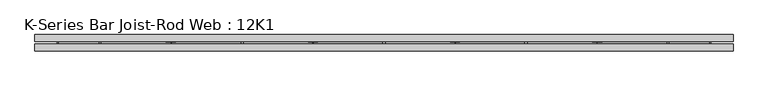
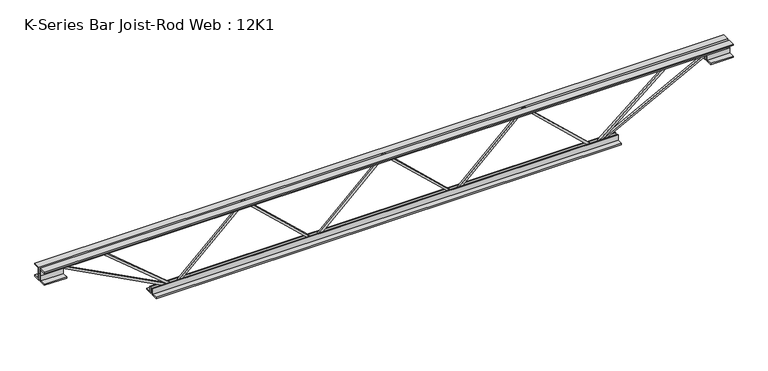
"""IFC4 building model written with IfcOpenShell, lengths in millimetres: beam geometry, K-Series Bar Joist-Rod Web : 12K1."""

from ifc_helpers import new_model, si_unit, frame, origin, place, context, project, spatial, polyline, outline, extrude, source, transform, mapped, element, save


def k_series_bar_joist_rod_web_12k1_26cdcae3(model_context):
    return source(origin(), model_context, "Body", "SweptSolid", [
        extrude(outline(polyline([(-141.2875, -318.29375), (-150.8125, -318.29375), (-150.8125, -313.2370636), (141.2875, -1.2933136), (141.2875, 1.2933136), (-150.8125, 313.2370636), (-150.8125, 318.29375), (-141.2875, 318.29375), (-141.2875, 317.0004364), (150.8125, 5.0566864), (150.8125, -5.0566864), (-141.2875, -317.0004364), (-141.2875, -318.29375)])), frame((0.0, -4.7625, 0.0), z_axis=(0.0, 1.0, 0.0), x_axis=(0.0, 0.0, 1.0)), (0.0, 0.0, 1.0), 9.525),
        extrude(outline(polyline([(-141.2875, 318.29375), (-150.8125, 318.29375), (-150.8125, 323.3504364), (141.2875, 635.2941864), (141.2875, 637.8808136), (-150.8125, 949.8245636), (-150.8125, 954.88125), (-141.2875, 954.88125), (-141.2875, 953.5879364), (150.8125, 641.6441864), (150.8125, 631.5308136), (-141.2875, 319.5870636), (-141.2875, 318.29375)])), frame((0.0, -4.7625, 0.0), z_axis=(0.0, 1.0, 0.0), x_axis=(0.0, 0.0, 1.0)), (0.0, 0.0, 1.0), 9.525),
        extrude(outline(polyline([(-141.2875, -954.88125), (-150.8125, -954.88125), (-150.8125, -949.8245636), (141.2875, -637.8808136), (141.2875, -635.2941864), (-150.8125, -323.3504364), (-150.8125, -318.29375), (-141.2875, -318.29375), (-141.2875, -319.5870636), (150.8125, -631.5308136), (150.8125, -641.6441864), (-141.2875, -953.5879364), (-141.2875, -954.88125)])), frame((0.0, -4.7625, 0.0), z_axis=(0.0, 1.0, 0.0), x_axis=(0.0, 0.0, 1.0)), (0.0, 0.0, 1.0), 9.525),
        extrude(outline(polyline([(4.7625, 152.4), (36.5125, 152.4), (36.5125, 146.05), (11.1125, 146.05), (11.1125, 120.65), (4.7625, 120.65), (4.7625, 152.4)])), frame((-1564.48125, 0.0, 0.0), z_axis=(1.0, 0.0, 0.0), x_axis=(0.0, 1.0, 0.0)), (0.0, 0.0, 1.0), 3128.9625),
        extrude(outline(polyline([(-4.7625, 152.4), (-4.7625, 120.65), (-11.1125, 120.65), (-11.1125, 146.05), (-36.5125, 146.05), (-36.5125, 152.4), (-4.7625, 152.4)])), frame((-1564.48125, 0.0, 0.0), z_axis=(1.0, 0.0, 0.0), x_axis=(0.0, 1.0, 0.0)), (0.0, 0.0, 1.0), 3128.9625),
        extrude(outline(polyline([(-4.7625, 88.9), (-36.5125, 88.9), (-36.5125, 95.25), (-11.1125, 95.25), (-11.1125, 120.65), (-4.7625, 120.65), (-4.7625, 88.9)])), frame((-1564.48125, 0.0, 0.0), z_axis=(1.0, 0.0, 0.0), x_axis=(0.0, 1.0, 0.0)), (0.0, 0.0, 1.0), 101.6),
        extrude(outline(polyline([(36.5125, 88.9), (4.7625, 88.9), (4.7625, 120.65), (11.1125, 120.65), (11.1125, 95.25), (36.5125, 95.25), (36.5125, 88.9)])), frame((-1564.48125, 0.0, 0.0), z_axis=(1.0, 0.0, 0.0), x_axis=(0.0, 1.0, 0.0)), (0.0, 0.0, 1.0), 101.6),
        extrude(outline(polyline([(4.7625, 88.9), (4.7625, 120.65), (11.1125, 120.65), (11.1125, 95.25), (36.5125, 95.25), (36.5125, 88.9), (4.7625, 88.9)])), frame((1462.88125, 0.0, 0.0), z_axis=(1.0, 0.0, 0.0), x_axis=(0.0, 1.0, 0.0)), (0.0, 0.0, 1.0), 101.6),
        extrude(outline(polyline([(-4.7625, 88.9), (-36.5125, 88.9), (-36.5125, 95.25), (-11.1125, 95.25), (-11.1125, 120.65), (-4.7625, 120.65), (-4.7625, 88.9)])), frame((1462.88125, 0.0, 0.0), z_axis=(1.0, 0.0, 0.0), x_axis=(0.0, 1.0, 0.0)), (0.0, 0.0, 1.0), 101.6),
        extrude(outline(polyline([(4.7625, -152.4), (4.7625, -120.65), (11.1125, -120.65), (11.1125, -146.05), (36.5125, -146.05), (36.5125, -152.4), (4.7625, -152.4)])), frame((-1056.48125, 0.0, 0.0), z_axis=(1.0, 0.0, 0.0), x_axis=(0.0, 1.0, 0.0)), (0.0, 0.0, 1.0), 2112.9625),
        extrude(outline(polyline([(-4.7625, -152.4), (-36.5125, -152.4), (-36.5125, -146.05), (-11.1125, -146.05), (-11.1125, -120.65), (-4.7625, -120.65), (-4.7625, -152.4)])), frame((-1056.48125, 0.0, 0.0), z_axis=(1.0, 0.0, 0.0), x_axis=(0.0, 1.0, 0.0)), (0.0, 0.0, 1.0), 2112.9625),
        extrude(outline(polyline([(0.0, -9.525), (0.0, 0.0), (573.7533355, 0.0), (573.7533355, -9.525), (0.0, -9.525)])), frame((-1465.0950214, 4.7625, 116.4332925), z_axis=(0.4648338989895144, 0.0, 0.8853979028381567), x_axis=(0.8853979028381567, 0.0, -0.4648338989895144)), (0.0, 0.0, 1.0), 9.525),
        extrude(outline(polyline([(0.0, -9.525), (0.0, 0.0), (415.2587161, 0.0), (415.2587161, -9.525), (0.0, -9.525)])), frame((-1276.2337167, 4.7625, 116.9995673), z_axis=(0.6422502157468647, 0.0, 0.766495049151073), x_axis=(0.766495049151073, 0.0, -0.6422502157468647)), (0.0, 0.0, 1.0), 9.525),
        extrude(outline(polyline([(0.0, -9.525), (0.0, 0.0), (573.7533355, 0.0), (573.7533355, -9.525), (0.0, -9.525)])), frame((1465.0950214, -4.7625, 116.4332925), z_axis=(-0.46483389898949484, 0.0, 0.885397902838167), x_axis=(-0.885397902838167, 0.0, -0.46483389898949484)), (0.0, 0.0, 1.0), 9.525),
        extrude(outline(polyline([(0.0, -9.525), (0.0, 0.0), (415.2587161, 0.0), (415.2587161, -9.525), (0.0, -9.525)])), frame((1276.2337167, -4.7625, 116.9995673), z_axis=(-0.6422502157468591, 0.0, 0.7664950491510777), x_axis=(-0.7664950491510777, 0.0, -0.6422502157468591)), (0.0, 0.0, 1.0), 9.525),
    ])


if __name__ == "__main__":
    model = new_model("IFC4")
    model_context = context("Model", 3, world=origin())
    ifc_project = project(units=[si_unit("LENGTHUNIT", "METRE", prefix="MILLI")], contexts=[model_context])
    site = spatial("IfcSite", under=ifc_project)
    building = spatial("IfcBuilding", under=site)
    placement = place(None, origin())
    k_series_bar_joist_rod_web_12k1_shape = k_series_bar_joist_rod_web_12k1_26cdcae3(model_context)
    element("IfcBeam", 1, ObjectType="K-Series Bar Joist-Rod Web : 12K1", at=placement, inside=building, context=model_context, shape_type="MappedRepresentation", body=[
        mapped(k_series_bar_joist_rod_web_12k1_shape, transform((0.0, 0.0, 0.0), x_axis=(1.0, 0.0, 0.0), y_axis=(0.0, 1.0, 0.0), z_axis=(0.0, 0.0, 1.0))),
    ])
    save(model, "model.ifc")

# Revit data of these elements
# Type "K-Series Bar Joist-Rod Web : 12K1"
#   Assembly Code = "B1010350"
#   Wt = 5
#   Web Thickness = 0' - 0 3/8"
#   Start Offset [instance default] = 0' - 0"
#   Start Extension [instance default] = 0' - 0"
#   Seat Length = 0' - 4"
#   Seat Depth = 0' - 2 1/2"
#   PanelArrayLength [instance default] = 20' - 0"
#   Panel [instance default] = 2' - 0"
#   End Offset [instance default] = 0' - 0"
#   End Extension [instance default] = 0' - 0"
#   End Panel = 2' - 0"
#   Cord Leg = 0' - 1 1/4"
#   Chord Thickness = 0' - 0 1/4"
#   Length [instance default] = 24' - 0"
#   Depth = 1' - 0"
#   PanelArrayNum [instance default] = 10
#   Structural Material = none
# Element 1 (IfcBeam, "K-Series Bar Joist-Rod Web : 12K1")
#   PanelArrayLength = 6' - 3 3/16"
#   Panel = 2' - 1 1/16"
#   PanelArrayNum = 3
